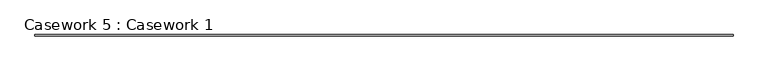
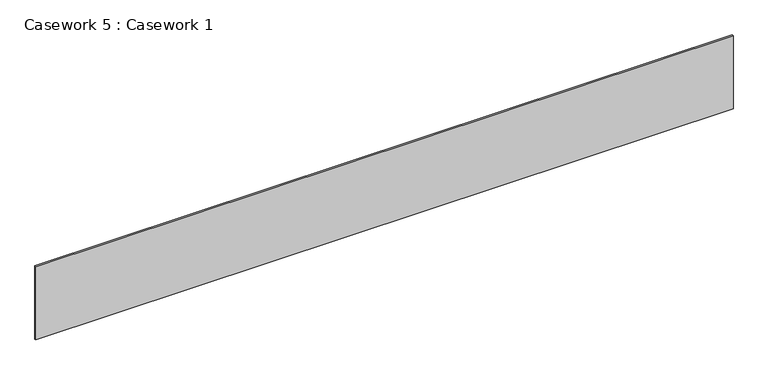
"""IFC4 building model written with IfcOpenShell, lengths in millimetres: furniture geometry, Casework 5 : Casework 1."""

from ifc_helpers import new_model, si_unit, frame, origin, place, context, project, spatial, polyline, outline, extrude, source, transform, mapped, element, save


def casework_5_casework_1_74b769df(model_context):
    return source(origin(), model_context, "Body", "SweptSolid", [
        extrude(outline(polyline([(-38619.6176606, 248021.3599557), (-50363.0431589, 248021.3599557), (-50363.0431589, 248046.7599557), (-38619.6176606, 248046.7599557), (-38619.6176606, 248021.3599557)])), frame((0.0, 0.0, 3340.1), z_axis=(0.0, 0.0, 1.0), x_axis=(1.0, 0.0, 0.0)), (0.0, 0.0, 1.0), 1303.445648),
    ])


if __name__ == "__main__":
    model = new_model("IFC4")
    model_context = context("Model", 3, world=origin())
    ifc_project = project(units=[si_unit("LENGTHUNIT", "METRE", prefix="MILLI")], contexts=[model_context])
    site = spatial("IfcSite", under=ifc_project)
    building = spatial("IfcBuilding", under=site)
    placement = place(None, origin())
    casework_5_casework_1_shape = casework_5_casework_1_74b769df(model_context)
    element("IfcFurniture", 1, ObjectType="Casework 5 : Casework 1", at=placement, inside=building, context=model_context, shape_type="MappedRepresentation", body=[
        mapped(casework_5_casework_1_shape, transform((0.0, 0.0, 0.0), x_axis=(1.0, 0.0, 0.0), y_axis=(0.0, 1.0, 0.0), z_axis=(0.0, 0.0, 1.0))),
    ])
    save(model, "model.ifc")

# Revit data of these elements
# Element 1 (IfcFurniture, "Casework 5 : Casework 1")
#   Materials on its faces: "METAL PANEL (DARK BRONZE) - TO MATCH MAIN BUILDING ACCENT METAL"
# Materials
#   "METAL PANEL (DARK BRONZE) - TO MATCH MAIN BUILDING ACCENT METAL": class "Generic", colour RGB 88 62 61, transparency 0, Cost = 0
